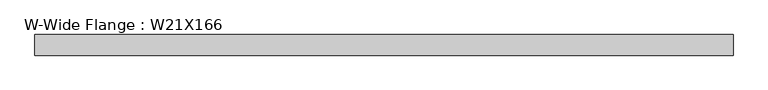
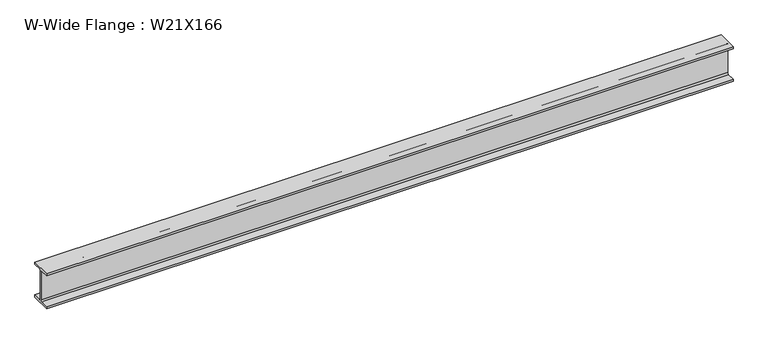
"""IFC4 building model written with IfcOpenShell, lengths in millimetres: beam geometry, W-Wide Flange : W21X166."""

import ifcopenshell
import ifcopenshell.guid

model = None  # the IFC model being written
_history = None  # IfcOwnerHistory: only IFC2X3 demands one
_inside = {}  # id of a spatial element -> (the spatial element, [elements in it])
_under = {}  # id of a project, library or spatial element -> (it, [spatial elements below it])
_declared = {}  # id of a project -> (the project, [libraries it declares])
_typed = {}  # id of a type object -> (the type object, [elements of that type])
_made_of = {}  # id of a material, layer set ... -> (it, [elements and type objects made of it])


def new_model(schema):
    """Start an empty IFC model of exactly this schema.

    Asked for "IFC4X3", IfcOpenShell would pick the latest addendum, in which some entities
    have other attributes; the version numbers below select the first issue.
    IFC2X3 requires an IfcOwnerHistory on every rooted entity: one is made here for all.
    """
    global model, _history
    if schema == "IFC4X3":
        model = ifcopenshell.file(schema_version=(4, 3, 0, 0))
    else:
        model = ifcopenshell.file(schema=schema)
    _inside.clear()
    _under.clear()
    _declared.clear()
    _typed.clear()
    _made_of.clear()
    _history = None
    if model.schema == "IFC2X3":
        org = make("IfcOrganization", Name="unknown")
        user = make(
            "IfcPersonAndOrganization",
            ThePerson=make("IfcPerson", FamilyName="unknown"),
            TheOrganization=org,
        )
        app = make(
            "IfcApplication",
            ApplicationDeveloper=org,
            Version="unknown",
            ApplicationFullName="unknown",
            ApplicationIdentifier="unknown",
        )
        _history = make(
            "IfcOwnerHistory",
            OwningUser=user,
            OwningApplication=app,
            ChangeAction="ADDED",
            CreationDate=0,
        )
    return model


def make(cls, **values):
    """One entity of the class cls with the attributes given. An attribute that is None is left unset."""
    return model.create_entity(
        cls, **{name: value for name, value in values.items() if value is not None}
    )


def rooted(cls, **values):
    """An entity with a GlobalId (a new one), such as an element, a storey or a relation."""
    return make(cls, GlobalId=ifcopenshell.guid.new(), OwnerHistory=_history, **values)


def si_unit(unit_type, name, prefix=None):
    """IfcSIUnit, for example si_unit("LENGTHUNIT", "METRE", prefix="MILLI")."""
    return make("IfcSIUnit", UnitType=unit_type, Prefix=prefix, Name=name)


def assignment(units):
    """IfcUnitAssignment: the units of a project."""
    return None if units is None else make("IfcUnitAssignment", Units=units)


def point(xyz):
    """IfcCartesianPoint."""
    return None if xyz is None else make("IfcCartesianPoint", Coordinates=xyz)


def direction(xyz):
    """IfcDirection."""
    return None if xyz is None else make("IfcDirection", DirectionRatios=xyz)


def frame(location, z_axis=None, x_axis=None):
    """IfcAxis2Placement3D, a coordinate frame: its origin and axes. An axis left out is left unset."""
    return make(
        "IfcAxis2Placement3D",
        Location=point(location),
        Axis=direction(z_axis),
        RefDirection=direction(x_axis),
    )


def frame_2d(location, x_axis=None):
    """IfcAxis2Placement2D, a coordinate frame in the plane: its origin and x axis."""
    return make(
        "IfcAxis2Placement2D", Location=point(location), RefDirection=direction(x_axis)
    )


def origin():
    """The frame at (0, 0, 0) with its axes left unset."""
    return frame((0.0, 0.0, 0.0))


def place(relative_to, where):
    """IfcLocalPlacement: puts the frame where relative to a parent placement (None: the world)."""
    return make(
        "IfcLocalPlacement", PlacementRelTo=relative_to, RelativePlacement=where
    )


def context(
    kind, dimensions, precision=None, world=None, true_north=None, identifier=None
):
    """IfcGeometricRepresentationContext, for example the 3D "Model" context."""
    return make(
        "IfcGeometricRepresentationContext",
        ContextIdentifier=identifier,
        ContextType=kind,
        CoordinateSpaceDimension=dimensions,
        Precision=precision,
        WorldCoordinateSystem=world,
        TrueNorth=true_north,
    )


def project(units=None, contexts=None):
    """IfcProject with its units and contexts."""
    return rooted(
        "IfcProject",
        Name="project",
        RepresentationContexts=contexts,
        UnitsInContext=assignment(units),
    )


def spatial(cls, under=None, at=None, **own):
    """A site, building, storey or space (cls), placed at a placement, below another one or the project."""
    s = rooted(cls, ObjectPlacement=at, **own)
    if under is not None:
        _under.setdefault(under.id(), (under, []))[1].append(s)
    return s


def polyline(points):
    """IfcPolyline through the points."""
    return make("IfcPolyline", Points=[point(p) for p in points])


def circle_curve(where, radius):
    """IfcCircle in the frame where."""
    return make("IfcCircle", Position=where, Radius=radius)


def trimmed(basis, trim1, trim2, sense, master):
    """IfcTrimmedCurve: the piece of a basis curve between two trims."""
    return make(
        "IfcTrimmedCurve",
        BasisCurve=basis,
        Trim1=trim1,
        Trim2=trim2,
        SenseAgreement=sense,
        MasterRepresentation=master,
    )


def segment(curve, same_sense, transition):
    """IfcCompositeCurveSegment."""
    return make(
        "IfcCompositeCurveSegment",
        Transition=transition,
        SameSense=same_sense,
        ParentCurve=curve,
    )


def composite_curve(segments, self_intersect=None):
    """IfcCompositeCurve: segments joined end to end."""
    return make("IfcCompositeCurve", Segments=segments, SelfIntersect=self_intersect)


def outline(outer, holes=None, kind="AREA"):
    """IfcArbitraryClosedProfileDef: a profile drawn as a closed curve; with holes, ...WithVoids."""
    if holes is None:
        return make("IfcArbitraryClosedProfileDef", ProfileType=kind, OuterCurve=outer)
    return make(
        "IfcArbitraryProfileDefWithVoids",
        ProfileType=kind,
        OuterCurve=outer,
        InnerCurves=holes,
    )


def extrude(swept, where, along, depth):
    """IfcExtrudedAreaSolid: the profile swept, set in the frame where, extruded along a direction by depth."""
    return make(
        "IfcExtrudedAreaSolid",
        SweptArea=swept,
        Position=where,
        ExtrudedDirection=direction(along),
        Depth=depth,
    )


def shape(context_of_items, identifier, shape_type, items):
    """IfcShapeRepresentation: the items that make up one representation, for example the "Body"."""
    return make(
        "IfcShapeRepresentation",
        ContextOfItems=context_of_items,
        RepresentationIdentifier=identifier,
        RepresentationType=shape_type,
        Items=items,
    )


def source(mapping_origin, context_of_items, identifier, shape_type, items):
    """IfcRepresentationMap: a shape defined once, which mapped items show again and again."""
    return make(
        "IfcRepresentationMap",
        MappingOrigin=mapping_origin,
        MappedRepresentation=shape(context_of_items, identifier, shape_type, items),
    )


def transform(
    local_origin,
    x_axis=None,
    y_axis=None,
    z_axis=None,
    scale=None,
    scale2=None,
    scale3=None,
    uniform=True,
):
    """IfcCartesianTransformationOperator3D, or its non-uniform kind. x_axis, y_axis, z_axis: its Axis1, 2, 3."""
    if uniform:
        return make(
            "IfcCartesianTransformationOperator3D",
            Axis1=direction(x_axis),
            Axis2=direction(y_axis),
            LocalOrigin=point(local_origin),
            Scale=scale,
            Axis3=direction(z_axis),
        )
    return make(
        "IfcCartesianTransformationOperator3DnonUniform",
        Axis1=direction(x_axis),
        Axis2=direction(y_axis),
        LocalOrigin=point(local_origin),
        Scale=scale,
        Axis3=direction(z_axis),
        Scale2=scale2,
        Scale3=scale3,
    )


def mapped(mapping_source, mapping_target):
    """IfcMappedItem: shows the shape of a source again, moved by a transform."""
    return make(
        "IfcMappedItem", MappingSource=mapping_source, MappingTarget=mapping_target
    )


def made_of(thing, what):
    """Note that an element or type object is made of a material, layer set ...; save() writes the relation."""
    if what is not None:
        _made_of.setdefault(what.id(), (what, []))[1].append(thing)
    return thing


def element(
    cls,
    number,
    at=None,
    inside=None,
    cuts=None,
    type_object=None,
    material=None,
    context=None,
    identifier="Body",
    shape_type=None,
    held_by="IfcProductDefinitionShape",
    body=None,
    shapes=None,
    **own,
):
    """One element of the class cls, such as IfcWall. Its Tag is "e" and its number.

    at: its placement. inside: the storey or other place that contains it. cuts: it is an
    opening in that element (IfcRelVoidsElement). A single representation is given by context,
    identifier, shape_type and body (its items); several are given by shapes. held_by: the class
    of the entity that holds the representations. save() writes the other relations.
    """
    e = rooted(cls, Tag="e%d" % number, ObjectPlacement=at, **own)
    if body is not None:
        shapes = [shape(context, identifier, shape_type, body)]
    if shapes is not None:
        e.Representation = make(held_by, Representations=shapes)
    if inside is not None:
        _inside.setdefault(inside.id(), (inside, []))[1].append(e)
    if cuts is not None:
        rooted(
            "IfcRelVoidsElement", RelatingBuildingElement=cuts, RelatedOpeningElement=e
        )
    if type_object is not None:
        _typed.setdefault(type_object.id(), (type_object, []))[1].append(e)
    return made_of(e, material)


def aggregate(whole, parts):
    """IfcRelAggregates: a whole, such as a stair, and the parts it consists of."""
    return rooted("IfcRelAggregates", RelatingObject=whole, RelatedObjects=parts)


def save(model, path):
    """Write the relations noted so far, then the file.

    IfcRelAggregates (storeys below a building ...), IfcRelContainedInSpatialStructure (elements
    in a storey), IfcRelDefinesByType, IfcRelAssociatesMaterial and IfcRelDeclares: one each for
    every whole, place, type object, material and project.
    """
    for whole, parts in _under.values():
        aggregate(whole, parts)
    for where, things in _inside.values():
        rooted(
            "IfcRelContainedInSpatialStructure",
            RelatedElements=things,
            RelatingStructure=where,
        )
    for kind, things in _typed.values():
        rooted("IfcRelDefinesByType", RelatedObjects=things, RelatingType=kind)
    for what, things in _made_of.values():
        rooted("IfcRelAssociatesMaterial", RelatedObjects=things, RelatingMaterial=what)
    for by, libraries in _declared.values():
        rooted("IfcRelDeclares", RelatingContext=by, RelatedDefinitions=libraries)
    model.write(path)


def w_wide_flange_w21x166_ceda09b2(model_context):
    return source(origin(), model_context, "Body", "SweptSolid", [
        extrude(outline(composite_curve([segment(polyline([(157.48, -251.206), (157.48, -285.75), (-157.48, -285.75), (-157.48, -251.206), (-32.131, -251.206)]), True, "CONTINUOUS"), segment(trimmed(circle_curve(frame_2d((-32.131, -228.6)), 22.606), [point((-32.131, -251.206))], [point((-9.525, -228.6))], True, "CARTESIAN"), True, "CONTINUOUS"), segment(polyline([(-9.525, -228.6), (-9.525, 228.6)]), True, "CONTINUOUS"), segment(trimmed(circle_curve(frame_2d((-32.131, 228.6)), 22.606), [point((-9.525, 228.6))], [point((-32.131, 251.206))], True, "CARTESIAN"), True, "CONTINUOUS"), segment(polyline([(-32.131, 251.206), (-157.48, 251.206), (-157.48, 285.75), (157.48, 285.75), (157.48, 251.206), (32.131, 251.206)]), True, "CONTINUOUS"), segment(trimmed(circle_curve(frame_2d((32.131, 228.6)), 22.606), [point((32.131, 251.206))], [point((9.525, 228.6))], True, "CARTESIAN"), True, "CONTINUOUS"), segment(polyline([(9.525, 228.6), (9.525, -228.6)]), True, "CONTINUOUS"), segment(trimmed(circle_curve(frame_2d((32.131, -228.6)), 22.606), [point((9.525, -228.6))], [point((32.131, -251.206))], True, "CARTESIAN"), True, "CONTINUOUS"), segment(polyline([(32.131, -251.206), (157.48, -251.206)]), True, "CONTINUOUS")], self_intersect=False)), frame((-5436.0857782, 0.0, 0.0), z_axis=(1.0, 0.0, 0.0), x_axis=(0.0, 1.0, 0.0)), (0.0, 0.0, 1.0), 10659.8214497),
    ])


if __name__ == "__main__":
    model = new_model("IFC4")
    model_context = context("Model", 3, world=origin())
    ifc_project = project(units=[si_unit("LENGTHUNIT", "METRE", prefix="MILLI")], contexts=[model_context])
    site = spatial("IfcSite", under=ifc_project)
    building = spatial("IfcBuilding", under=site)
    placement = place(None, origin())
    w_wide_flange_w21x166_shape = w_wide_flange_w21x166_ceda09b2(model_context)
    element("IfcBeam", 1, ObjectType="W-Wide Flange : W21X166", at=placement, inside=building, context=model_context, shape_type="MappedRepresentation", body=[
        mapped(w_wide_flange_w21x166_shape, transform((0.0, 0.0, 0.0), x_axis=(1.0, 0.0, 0.0), y_axis=(0.0, 1.0, 0.0), z_axis=(0.0, 0.0, 1.0))),
    ])
    save(model, "model.ifc")

# Revit data of these elements
# Type "W-Wide Flange : W21X166"
#   Assembly Code = "B10"
#   W = 166
#   Length [instance default] = 5' - 0"
#   bf = 1' - 0.4"
#   d = 1' - 10 1/2"
#   k = 0' - 2 1/4"
#   k2 = 0' - 0.89"
#   tf = 0' - 1.36"
#   tw = 0' - 0 3/4"
#   A = 0.338889 SF
#   Structural Material [instance default] = Steel ASTM A992
# Element 1 (IfcBeam, "W-Wide Flange : W21X166")
#   Structural Material = Steel
#   Materials on its faces: "Steel"
# Materials
#   "Steel ASTM A992": class "Metal", colour RGB 199 199 199, transparency 0, Description = "Structural steel 50ksi", Cost = 0
#   "Steel": class "Metal", colour RGB 118 118 114, transparency 0, Description = "Steel, mill finish", Cost = 0
